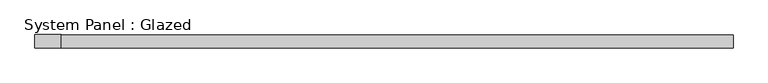
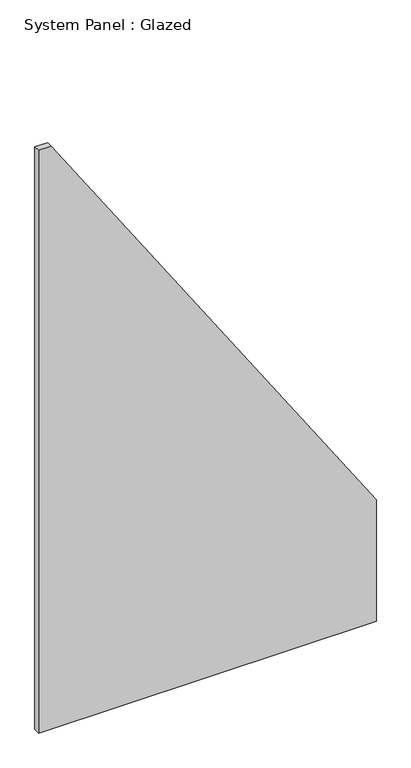
"""IFC4 building model written with IfcOpenShell, lengths in millimetres: plate geometry, System Panel : Glazed."""

from ifc_helpers import new_model, si_unit, frame, origin, place, context, project, spatial, polyline, outline, extrude, source, transform, mapped, element, save


def system_panel_glazed_b88468c6(model_context):
    return source(origin(), model_context, "Body", "SweptSolid", [
        extrude(outline(polyline([(0.0, -658.3333333), (0.0, 658.3333333), (499.353934, 658.3333333), (2400.0, -608.9382443), (2400.0, -658.3333333), (0.0, -658.3333333)])), frame((0.0, 24.5, 0.0), z_axis=(0.0, 1.0, 0.0), x_axis=(0.0, 0.0, 1.0)), (0.0, 0.0, 1.0), 25.0),
    ])


if __name__ == "__main__":
    model = new_model("IFC4")
    model_context = context("Model", 3, world=origin())
    ifc_project = project(units=[si_unit("LENGTHUNIT", "METRE", prefix="MILLI")], contexts=[model_context])
    site = spatial("IfcSite", under=ifc_project)
    building = spatial("IfcBuilding", under=site)
    placement = place(None, origin())
    system_panel_glazed_shape = system_panel_glazed_b88468c6(model_context)
    element("IfcPlate", 1, ObjectType="System Panel : Glazed", at=placement, inside=building, context=model_context, shape_type="MappedRepresentation", body=[
        mapped(system_panel_glazed_shape, transform((0.0, 0.0, 0.0), x_axis=(1.0, 0.0, 0.0), y_axis=(0.0, 1.0, 0.0), z_axis=(0.0, 0.0, 1.0))),
    ])
    save(model, "model.ifc")

# Revit data of these elements
# Type "System Panel : Glazed"
#   Keynote = "H11"
#   Construction Type Id = "GSP4R"
#   Analytic Construction = "1/8 in Pilkington single glazing"
#   Visual Light Transmittance = 0.9
#   Solar Heat Gain Coefficient = 0.86
#   Heat Transfer Coefficient (U) = 6.7069 W/(m²·K)
#   Define Thermal Properties by = 1
# Element 1 (IfcPlate, "System Panel : Glazed")
#   Materials on its faces: "Glass"
# Materials
#   "Glass": class "Glass", colour RGB 0 128 192, transparency 0.9, Description = "Soda Lime Glass", Cost = 0
